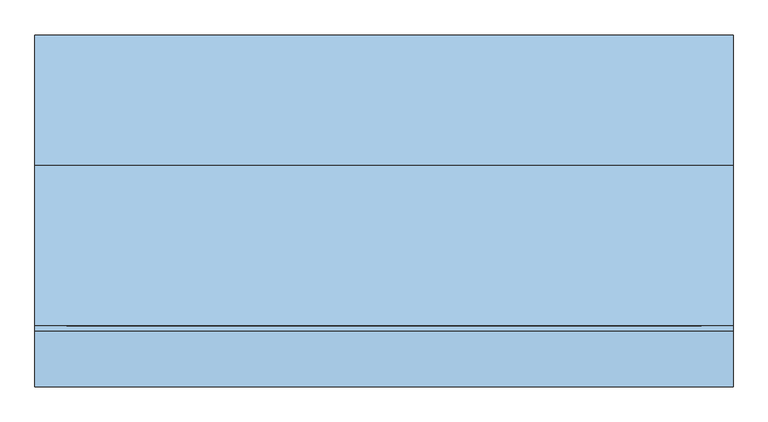
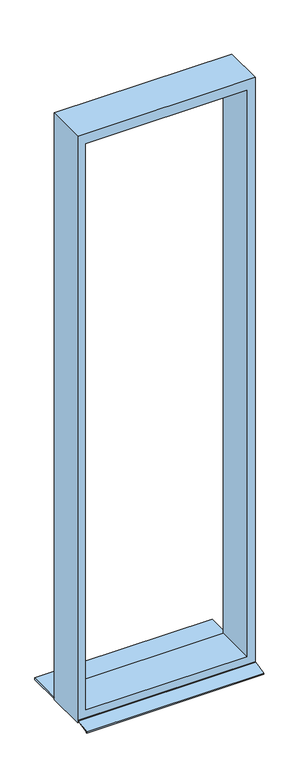
"""IFC4 building model written with IfcOpenShell, lengths in millimetres: window geometry, Fenster - Festverglasung : Feste Verglasung 4.58 x 1.31 3 2 2."""

from ifc_helpers import new_model, si_unit, frame, origin, place, context, project, spatial, polyline, outline, extrude, source, transform, mapped, element, save


def window_f6c59177(model_context):
    return source(origin(), model_context, "Body", "SweptSolid", [
        extrude(outline(polyline([(5580.0, 655.0), (5580.0, -655.0), (1000.0, -655.0), (1000.0, 655.0), (5580.0, 655.0)]), holes=[polyline([(5500.0, 595.0), (1080.0, 595.0), (1080.0, -595.0), (5500.0, -595.0), (5500.0, 595.0)])]), frame((0.0, -215.8682116, 0.0), z_axis=(0.0, 1.0, 0.0), x_axis=(0.0, 0.0, 1.0)), (0.0, 0.0, 1.0), 300.0),
        extrude(outline(polyline([(-655.0, 330.0), (655.0, 330.0), (655.0, 84.1317884), (-655.0, 84.1317884), (-655.0, 330.0)])), frame((0.0, 0.0, 1005.0), z_axis=(0.0, 0.0, 1.0), x_axis=(1.0, 0.0, 0.0)), (0.0, 0.0, 1.0), 15.0),
        extrude(outline(polyline([(-225.8903659, 1020.0), (-215.8682116, 1020.0), (-215.8682116, 1018.0), (-225.6922839, 1018.0), (-328.0, 998.3604634), (-328.0, 990.0), (-330.0, 990.0), (-330.0, 1000.0), (-225.8903659, 1020.0)])), frame((-655.0, 0.0, 0.0), z_axis=(1.0, 0.0, 0.0), x_axis=(0.0, 1.0, 0.0)), (0.0, 0.0, 1.0), 1310.0),
    ])


if __name__ == "__main__":
    model = new_model("IFC4")
    model_context = context("Model", 3, world=origin())
    ifc_project = project(units=[si_unit("LENGTHUNIT", "METRE", prefix="MILLI")], contexts=[model_context])
    site = spatial("IfcSite", under=ifc_project)
    building = spatial("IfcBuilding", under=site)
    placement = place(None, origin())
    window_shape = window_f6c59177(model_context)
    element("IfcWindow", 1, ObjectType="Fenster - Festverglasung : Feste Verglasung 4.58 x 1.31 3 2 2", at=placement, inside=building, context=model_context, shape_type="MappedRepresentation", body=[
        mapped(window_shape, transform((0.0, 0.0, 0.0), x_axis=(1.0, 0.0, 0.0), y_axis=(0.0, 1.0, 0.0), z_axis=(0.0, 0.0, 1.0))),
    ])
    save(model, "model.ifc")

# Revit data of these elements
# Type "Fenster - Festverglasung : Feste Verglasung 4.58 x 1.31 3 2 2"
#   Type Mark = "63"
#   Operation = "SinglePanel"
#   Keynote = "16.05.01"
#   Visual Light Transmittance = 0.9
#   Solar Heat Gain Coefficient = 0.78
#   Rough Width = 1.310 m
#   Rough Height = 4.580 m
#   Heat Transfer Coefficient (U) = 3.6886 W/(m²·K)
#   Rahmentiefe = 0.300 m
#   Rahmenhöhe unten = 0.080 m
#   Höhe oberer  Rahmen = 0.080 m
#   Rahmenbreite = 0.060 m
#   Height = 4.580 m
#   Einbautiefe (von außen) [instance default] = 0.080 m
#   Width = 1.310 m
#   Wall Closure = 3
#   Bild [instance default] = none
#   Glas [instance default] = none
#   Innere Fensterbank [instance default] = none
#   Äußere Fensterbank [instance default] = none
#   Construction Type Id = ""
#   Analytic Construction = (empty or 0)
# Element 1 (IfcWindow, "Fenster - Festverglasung : Feste Verglasung 4.58 x 1.31 3 2 2")
#   Einbautiefe (von außen) = 0.084132 m
#   Materials on its faces: "Kunststoff - Weiß", "Holz - Birke"
# Materials
#   "Kunststoff - Weiß": class "Kunststoff", colour RGB 249 249 249, transparency 0, Cost = 0
#   "Holz - Birke": class "Holz", colour RGB 213 164 103, transparency 0, Cost = 0
